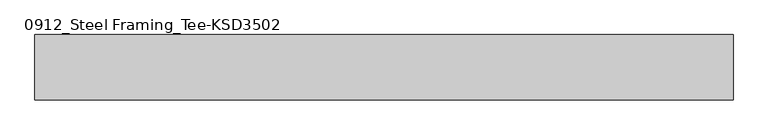
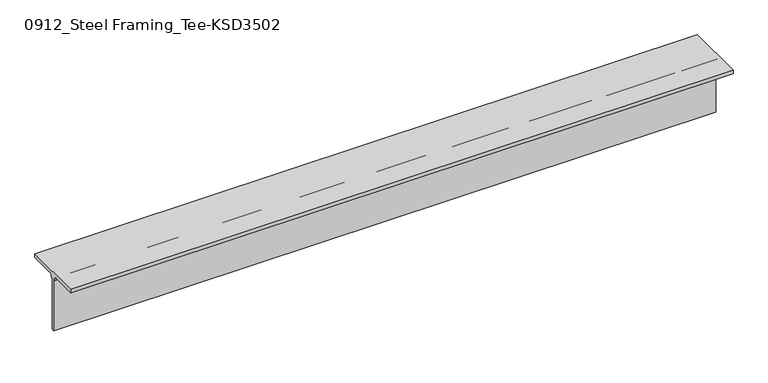
"""IFC4 building model written with IfcOpenShell, lengths in millimetres: member geometry, 0912_Steel Framing_Tee-KSD3502 : H_SB_ASB_CT-150x150x6.5x9."""

from ifc_helpers import new_model, si_unit, point, frame, frame_2d, origin, place, context, project, spatial, polyline, circle_curve, trimmed, segment, composite_curve, outline, extrude, source, transform, mapped, element, save


def member_0912_steel_framing_tee_ksd3502_15701a3e(model_context):
    return source(origin(), model_context, "Body", "SweptSolid", [
        extrude(outline(composite_curve([segment(polyline([(-75.0, 75.0), (75.0, 75.0), (75.0, 66.0), (16.25, 66.0)]), True, "CONTINUOUS"), segment(trimmed(circle_curve(frame_2d((16.25, 53.0)), 13.0), [point((16.25, 66.0))], [point((3.25, 53.0))], True, "CARTESIAN"), True, "CONTINUOUS"), segment(polyline([(3.25, 53.0), (3.25, -75.0), (-3.25, -75.0), (-3.25, 53.0)]), True, "CONTINUOUS"), segment(trimmed(circle_curve(frame_2d((-16.25, 53.0)), 13.0), [point((-3.25, 53.0))], [point((-16.25, 66.0))], True, "CARTESIAN"), True, "CONTINUOUS"), segment(polyline([(-16.25, 66.0), (-75.0, 66.0), (-75.0, 75.0)]), True, "CONTINUOUS")], self_intersect=False)), frame((-983.95, 0.0, 0.0), z_axis=(1.0, 0.0, 0.0), x_axis=(0.0, 1.0, 0.0)), (0.0, 0.0, 1.0), 1603.8),
    ])


if __name__ == "__main__":
    model = new_model("IFC4")
    model_context = context("Model", 3, world=origin())
    ifc_project = project(units=[si_unit("LENGTHUNIT", "METRE", prefix="MILLI")], contexts=[model_context])
    site = spatial("IfcSite", under=ifc_project)
    building = spatial("IfcBuilding", under=site)
    placement = place(None, origin())
    member_0912_steel_framing_tee_ksd3502_shape = member_0912_steel_framing_tee_ksd3502_15701a3e(model_context)
    element("IfcMember", 1, ObjectType="0912_Steel Framing_Tee-KSD3502 : H_SB_ASB_CT-150x150x6.5x9", at=placement, inside=building, context=model_context, shape_type="MappedRepresentation", body=[
        mapped(member_0912_steel_framing_tee_ksd3502_shape, transform((0.0, 0.0, 0.0), x_axis=(1.0, 0.0, 0.0), y_axis=(0.0, 1.0, 0.0), z_axis=(0.0, 0.0, 1.0))),
    ])
    save(model, "model.ifc")

# Revit data of these elements
# Type "0912_Steel Framing_Tee-KSD3502 : H_SB_ASB_CT-150x150x6.5x9"
#   H_WM Code_1 = "S01AA003-00001 | Main Steel Structure Fabrication Work | Shelter/Building | Light Steel - Standard (30KG/M>Weight) | Material: (   )"
#   H_WM Code_2 = "S03AA029-00001 | Main Steel Structure Erection Work | Shelter/Building | Light Steel (30KG/M>Weight) | Material: (   )"
#   H_WM Code_3 = "S01AA010-00001 | Main Steel Structure Fabrication Work | Shelter/Building | Steel Painting/Coating | for Non-Fireproofed Steel Surface, Surface Preparation, Primer, Second & Final Coat | Material: (   )"
#   H_Q'ty Cal Type Tag = "SB-Q2"
#   Width = 15.0 cm
#   Web Thickness = 0.65 cm
#   Web Fillet = 1.3 cm
#   Section Area = 23.39 cm²
#   Perimeter = 0.60 m²/m
#   Nominal Weight = 18.40 kgf/m
#   Height = 15.0 cm
#   Flange Thickness = 0.9 cm
#   Centroid Vertical = 7.5 cm
#   Centroid Horizontal = 7.5 cm
#   Length [instance default] = 1.5000 m
#   Structural Material [instance default] = Steel, 45-345
#   Warping Constant = (empty or 0)
#   Torsional Moment of Inertia = 0
#   Section Name Key = ""
#   Plastic Modulus weak axis = 0
#   Plastic Modulus strong axis = 0
#   Moment of Inertia weak axis = 0
#   Moment of Inertia strong axis = 0
#   Elastic Modulus weak axis = 0
#   Elastic Modulus strong axis = 0
#   Bolt Spacing = 0
#   Assembly Code = ""
# Element 1 (IfcMember, "0912_Steel Framing_Tee-KSD3502 : H_SB_ASB_CT-150x150x6.5x9")
#   Structural Material = none
# Materials
#   "Steel, 45-345": class "Metal", colour RGB 189 187 185, transparency 0, Description = "Steel 345 MPa", Cost = 0
